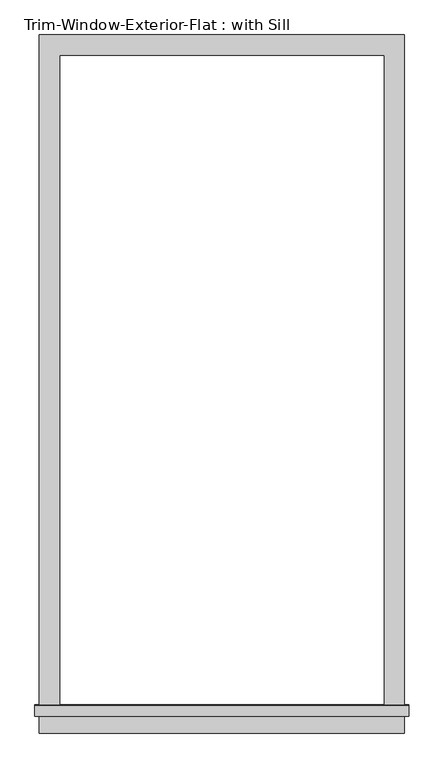
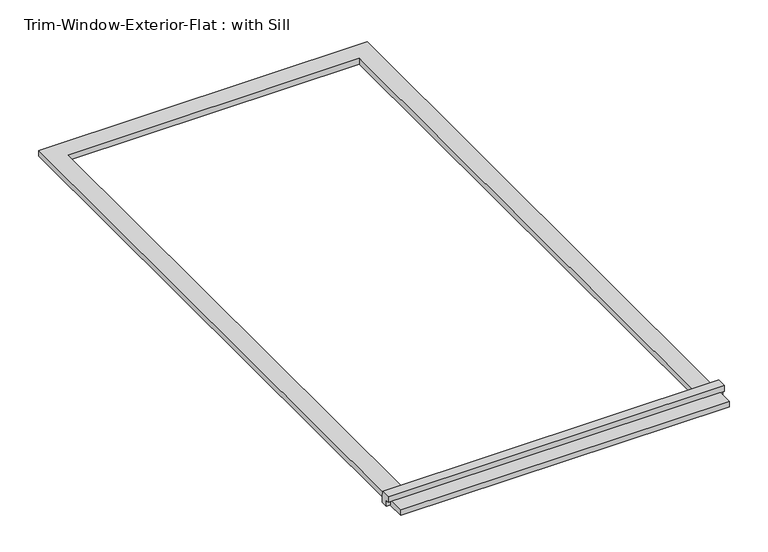
"""IFC4 building model written with IfcOpenShell, lengths in millimetres: proxy geometry, Trim-Window-Exterior-Flat : with Sill."""

import ifcopenshell
import ifcopenshell.guid

model = None  # the IFC model being written
_history = None  # IfcOwnerHistory: only IFC2X3 demands one
_inside = {}  # id of a spatial element -> (the spatial element, [elements in it])
_under = {}  # id of a project, library or spatial element -> (it, [spatial elements below it])
_declared = {}  # id of a project -> (the project, [libraries it declares])
_typed = {}  # id of a type object -> (the type object, [elements of that type])
_made_of = {}  # id of a material, layer set ... -> (it, [elements and type objects made of it])


def new_model(schema):
    """Start an empty IFC model of exactly this schema.

    Asked for "IFC4X3", IfcOpenShell would pick the latest addendum, in which some entities
    have other attributes; the version numbers below select the first issue.
    IFC2X3 requires an IfcOwnerHistory on every rooted entity: one is made here for all.
    """
    global model, _history
    if schema == "IFC4X3":
        model = ifcopenshell.file(schema_version=(4, 3, 0, 0))
    else:
        model = ifcopenshell.file(schema=schema)
    _inside.clear()
    _under.clear()
    _declared.clear()
    _typed.clear()
    _made_of.clear()
    _history = None
    if model.schema == "IFC2X3":
        org = make("IfcOrganization", Name="unknown")
        user = make(
            "IfcPersonAndOrganization",
            ThePerson=make("IfcPerson", FamilyName="unknown"),
            TheOrganization=org,
        )
        app = make(
            "IfcApplication",
            ApplicationDeveloper=org,
            Version="unknown",
            ApplicationFullName="unknown",
            ApplicationIdentifier="unknown",
        )
        _history = make(
            "IfcOwnerHistory",
            OwningUser=user,
            OwningApplication=app,
            ChangeAction="ADDED",
            CreationDate=0,
        )
    return model


def make(cls, **values):
    """One entity of the class cls with the attributes given. An attribute that is None is left unset."""
    return model.create_entity(
        cls, **{name: value for name, value in values.items() if value is not None}
    )


def rooted(cls, **values):
    """An entity with a GlobalId (a new one), such as an element, a storey or a relation."""
    return make(cls, GlobalId=ifcopenshell.guid.new(), OwnerHistory=_history, **values)


def si_unit(unit_type, name, prefix=None):
    """IfcSIUnit, for example si_unit("LENGTHUNIT", "METRE", prefix="MILLI")."""
    return make("IfcSIUnit", UnitType=unit_type, Prefix=prefix, Name=name)


def assignment(units):
    """IfcUnitAssignment: the units of a project."""
    return None if units is None else make("IfcUnitAssignment", Units=units)


def point(xyz):
    """IfcCartesianPoint."""
    return None if xyz is None else make("IfcCartesianPoint", Coordinates=xyz)


def direction(xyz):
    """IfcDirection."""
    return None if xyz is None else make("IfcDirection", DirectionRatios=xyz)


def frame(location, z_axis=None, x_axis=None):
    """IfcAxis2Placement3D, a coordinate frame: its origin and axes. An axis left out is left unset."""
    return make(
        "IfcAxis2Placement3D",
        Location=point(location),
        Axis=direction(z_axis),
        RefDirection=direction(x_axis),
    )


def origin():
    """The frame at (0, 0, 0) with its axes left unset."""
    return frame((0.0, 0.0, 0.0))


def origin_with_axes():
    """The frame at (0, 0, 0) with the z axis (0, 0, 1) and the x axis (1, 0, 0) written out."""
    return frame((0.0, 0.0, 0.0), z_axis=(0.0, 0.0, 1.0), x_axis=(1.0, 0.0, 0.0))


def place(relative_to, where):
    """IfcLocalPlacement: puts the frame where relative to a parent placement (None: the world)."""
    return make(
        "IfcLocalPlacement", PlacementRelTo=relative_to, RelativePlacement=where
    )


def context(
    kind, dimensions, precision=None, world=None, true_north=None, identifier=None
):
    """IfcGeometricRepresentationContext, for example the 3D "Model" context."""
    return make(
        "IfcGeometricRepresentationContext",
        ContextIdentifier=identifier,
        ContextType=kind,
        CoordinateSpaceDimension=dimensions,
        Precision=precision,
        WorldCoordinateSystem=world,
        TrueNorth=true_north,
    )


def project(units=None, contexts=None):
    """IfcProject with its units and contexts."""
    return rooted(
        "IfcProject",
        Name="project",
        RepresentationContexts=contexts,
        UnitsInContext=assignment(units),
    )


def spatial(cls, under=None, at=None, **own):
    """A site, building, storey or space (cls), placed at a placement, below another one or the project."""
    s = rooted(cls, ObjectPlacement=at, **own)
    if under is not None:
        _under.setdefault(under.id(), (under, []))[1].append(s)
    return s


def polyline(points):
    """IfcPolyline through the points."""
    return make("IfcPolyline", Points=[point(p) for p in points])


def outline(outer, holes=None, kind="AREA"):
    """IfcArbitraryClosedProfileDef: a profile drawn as a closed curve; with holes, ...WithVoids."""
    if holes is None:
        return make("IfcArbitraryClosedProfileDef", ProfileType=kind, OuterCurve=outer)
    return make(
        "IfcArbitraryProfileDefWithVoids",
        ProfileType=kind,
        OuterCurve=outer,
        InnerCurves=holes,
    )


def extrude(swept, where, along, depth):
    """IfcExtrudedAreaSolid: the profile swept, set in the frame where, extruded along a direction by depth."""
    return make(
        "IfcExtrudedAreaSolid",
        SweptArea=swept,
        Position=where,
        ExtrudedDirection=direction(along),
        Depth=depth,
    )


def shape(context_of_items, identifier, shape_type, items):
    """IfcShapeRepresentation: the items that make up one representation, for example the "Body"."""
    return make(
        "IfcShapeRepresentation",
        ContextOfItems=context_of_items,
        RepresentationIdentifier=identifier,
        RepresentationType=shape_type,
        Items=items,
    )


def source(mapping_origin, context_of_items, identifier, shape_type, items):
    """IfcRepresentationMap: a shape defined once, which mapped items show again and again."""
    return make(
        "IfcRepresentationMap",
        MappingOrigin=mapping_origin,
        MappedRepresentation=shape(context_of_items, identifier, shape_type, items),
    )


def transform(
    local_origin,
    x_axis=None,
    y_axis=None,
    z_axis=None,
    scale=None,
    scale2=None,
    scale3=None,
    uniform=True,
):
    """IfcCartesianTransformationOperator3D, or its non-uniform kind. x_axis, y_axis, z_axis: its Axis1, 2, 3."""
    if uniform:
        return make(
            "IfcCartesianTransformationOperator3D",
            Axis1=direction(x_axis),
            Axis2=direction(y_axis),
            LocalOrigin=point(local_origin),
            Scale=scale,
            Axis3=direction(z_axis),
        )
    return make(
        "IfcCartesianTransformationOperator3DnonUniform",
        Axis1=direction(x_axis),
        Axis2=direction(y_axis),
        LocalOrigin=point(local_origin),
        Scale=scale,
        Axis3=direction(z_axis),
        Scale2=scale2,
        Scale3=scale3,
    )


def mapped(mapping_source, mapping_target):
    """IfcMappedItem: shows the shape of a source again, moved by a transform."""
    return make(
        "IfcMappedItem", MappingSource=mapping_source, MappingTarget=mapping_target
    )


def made_of(thing, what):
    """Note that an element or type object is made of a material, layer set ...; save() writes the relation."""
    if what is not None:
        _made_of.setdefault(what.id(), (what, []))[1].append(thing)
    return thing


def element(
    cls,
    number,
    at=None,
    inside=None,
    cuts=None,
    type_object=None,
    material=None,
    context=None,
    identifier="Body",
    shape_type=None,
    held_by="IfcProductDefinitionShape",
    body=None,
    shapes=None,
    **own,
):
    """One element of the class cls, such as IfcWall. Its Tag is "e" and its number.

    at: its placement. inside: the storey or other place that contains it. cuts: it is an
    opening in that element (IfcRelVoidsElement). A single representation is given by context,
    identifier, shape_type and body (its items); several are given by shapes. held_by: the class
    of the entity that holds the representations. save() writes the other relations.
    """
    e = rooted(cls, Tag="e%d" % number, ObjectPlacement=at, **own)
    if body is not None:
        shapes = [shape(context, identifier, shape_type, body)]
    if shapes is not None:
        e.Representation = make(held_by, Representations=shapes)
    if inside is not None:
        _inside.setdefault(inside.id(), (inside, []))[1].append(e)
    if cuts is not None:
        rooted(
            "IfcRelVoidsElement", RelatingBuildingElement=cuts, RelatedOpeningElement=e
        )
    if type_object is not None:
        _typed.setdefault(type_object.id(), (type_object, []))[1].append(e)
    return made_of(e, material)


def aggregate(whole, parts):
    """IfcRelAggregates: a whole, such as a stair, and the parts it consists of."""
    return rooted("IfcRelAggregates", RelatingObject=whole, RelatedObjects=parts)


def save(model, path):
    """Write the relations noted so far, then the file.

    IfcRelAggregates (storeys below a building ...), IfcRelContainedInSpatialStructure (elements
    in a storey), IfcRelDefinesByType, IfcRelAssociatesMaterial and IfcRelDeclares: one each for
    every whole, place, type object, material and project.
    """
    for whole, parts in _under.values():
        aggregate(whole, parts)
    for where, things in _inside.values():
        rooted(
            "IfcRelContainedInSpatialStructure",
            RelatedElements=things,
            RelatingStructure=where,
        )
    for kind, things in _typed.values():
        rooted("IfcRelDefinesByType", RelatedObjects=things, RelatingType=kind)
    for what, things in _made_of.values():
        rooted("IfcRelAssociatesMaterial", RelatedObjects=things, RelatingMaterial=what)
    for by, libraries in _declared.values():
        rooted("IfcRelDeclares", RelatingContext=by, RelatedDefinitions=libraries)
    model.write(path)


def trim_window_exterior_flat_with_sill_c2ca58d6(model_context):
    return source(origin(), model_context, "Body", "SweptSolid", [
        extrude(outline(polyline([(514.35, -1850.9823709), (514.35, -1908.1323709), (-514.35, -1908.1323709), (-514.35, -1850.9823709), (514.35, -1850.9823709)])), origin_with_axes(), (0.0, 0.0, 1.0), 19.05),
        extrude(outline(polyline([(-1860.55, 38.1), (-1831.2580645, 38.1), (-1828.8, 19.05), (-1828.8, 0.0), (-1850.9823709, 0.0), (-1850.9823709, 19.05), (-1860.55, 19.05), (-1860.55, 38.1)])), frame((-527.05, 0.0, 0.0), z_axis=(1.0, 0.0, 0.0), x_axis=(0.0, 1.0, 0.0)), (0.0, 0.0, 1.0), 1054.1),
        extrude(outline(polyline([(-514.35, 57.15), (514.35, 57.15), (514.35, -1828.8), (457.2, -1828.8), (457.2, 0.0), (-457.2, 0.0), (-457.2, -1828.8), (-514.35, -1828.8), (-514.35, 57.15)])), origin_with_axes(), (0.0, 0.0, 1.0), 19.05),
    ])


if __name__ == "__main__":
    model = new_model("IFC4")
    model_context = context("Model", 3, world=origin())
    ifc_project = project(units=[si_unit("LENGTHUNIT", "METRE", prefix="MILLI")], contexts=[model_context])
    site = spatial("IfcSite", under=ifc_project)
    building = spatial("IfcBuilding", under=site)
    placement = place(None, origin())
    trim_window_exterior_flat_with_sill_shape = trim_window_exterior_flat_with_sill_c2ca58d6(model_context)
    element("IfcBuildingElementProxy", 1, Name="Trim-Window-Exterior-Flat : with Sill", ObjectType="Trim-Window-Exterior-Flat : with Sill", at=placement, inside=building, context=model_context, shape_type="MappedRepresentation", body=[
        mapped(trim_window_exterior_flat_with_sill_shape, transform((0.0, 0.0, 0.0), x_axis=(1.0, 0.0, 0.0), y_axis=(0.0, 1.0, 0.0), z_axis=(0.0, 0.0, 1.0))),
    ])
    save(model, "model.ifc")

# Revit data of these elements
# Type "Trim-Window-Exterior-Flat : with Sill"
#   Trim Width = 0' - 2 1/4"
#   Trim Thickness_Picture Frame = 0' - 1 1/4"
#   Trim Thickness_with Sill = 0' - 0 3/4"
#   Sill Thickness = 0' - 1 1/4"
#   Opening Width [instance default] = 2' - 0"
#   Opening Height [instance default] = 3' - 0"
#   Default Elevation = 4' - 0"
#   Sill = yes
#   Picture Frame = no
#   Trim Material [instance default] = none
# Element 1 (IfcBuildingElementProxy, "Trim-Window-Exterior-Flat : with Sill")
#   Opening Width = 3' - 0"
#   Opening Height = 6' - 0"
#   Trim Material = Clad - White
#   Materials on its faces: "Clad - White"
# Materials
#   "Clad - White": class "Wood", colour RGB 242 242 238, transparency 0, Cost = 0
